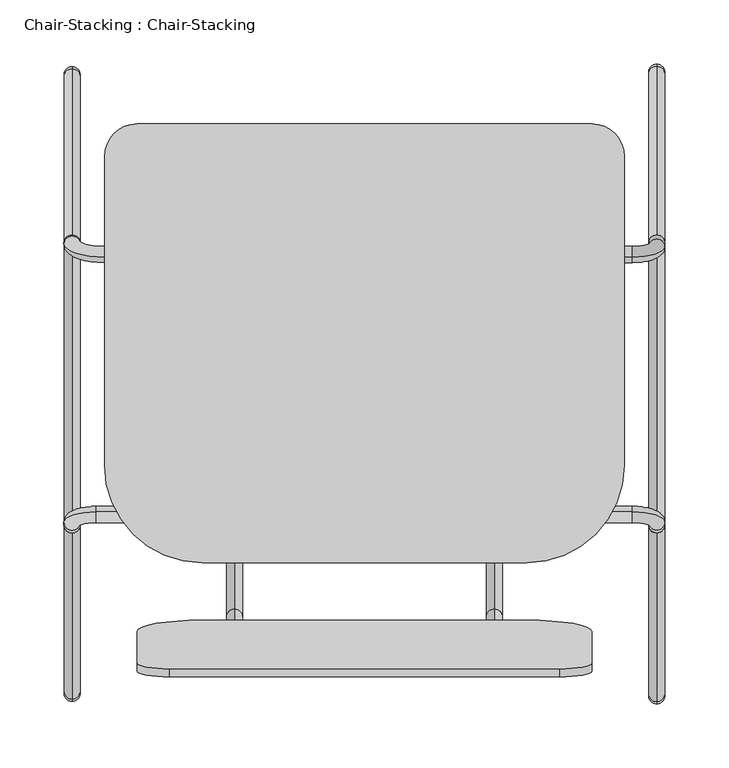
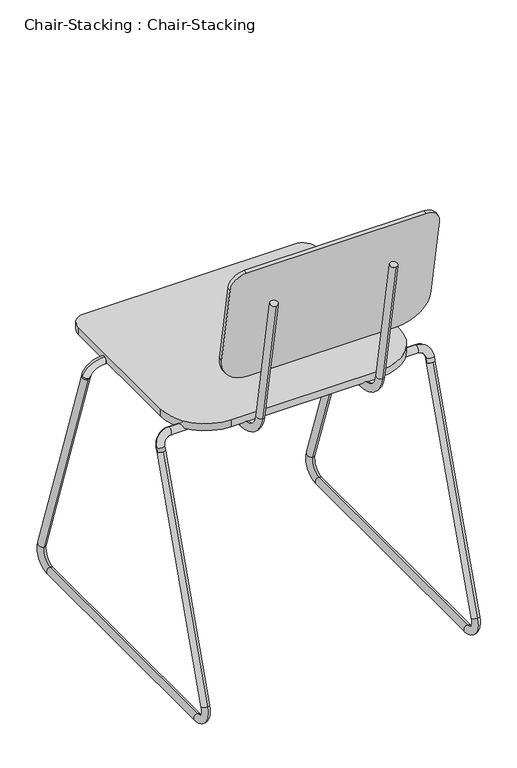
"""IFC4 building model written with IfcOpenShell, lengths in millimetres: furniture geometry, Chair-Stacking : Chair-Stacking."""

import ifcopenshell
import ifcopenshell.guid

model = None  # the IFC model being written
_history = None  # IfcOwnerHistory: only IFC2X3 demands one
_inside = {}  # id of a spatial element -> (the spatial element, [elements in it])
_under = {}  # id of a project, library or spatial element -> (it, [spatial elements below it])
_declared = {}  # id of a project -> (the project, [libraries it declares])
_typed = {}  # id of a type object -> (the type object, [elements of that type])
_made_of = {}  # id of a material, layer set ... -> (it, [elements and type objects made of it])


def new_model(schema):
    """Start an empty IFC model of exactly this schema.

    Asked for "IFC4X3", IfcOpenShell would pick the latest addendum, in which some entities
    have other attributes; the version numbers below select the first issue.
    IFC2X3 requires an IfcOwnerHistory on every rooted entity: one is made here for all.
    """
    global model, _history
    if schema == "IFC4X3":
        model = ifcopenshell.file(schema_version=(4, 3, 0, 0))
    else:
        model = ifcopenshell.file(schema=schema)
    _inside.clear()
    _under.clear()
    _declared.clear()
    _typed.clear()
    _made_of.clear()
    _history = None
    if model.schema == "IFC2X3":
        org = make("IfcOrganization", Name="unknown")
        user = make(
            "IfcPersonAndOrganization",
            ThePerson=make("IfcPerson", FamilyName="unknown"),
            TheOrganization=org,
        )
        app = make(
            "IfcApplication",
            ApplicationDeveloper=org,
            Version="unknown",
            ApplicationFullName="unknown",
            ApplicationIdentifier="unknown",
        )
        _history = make(
            "IfcOwnerHistory",
            OwningUser=user,
            OwningApplication=app,
            ChangeAction="ADDED",
            CreationDate=0,
        )
    return model


def make(cls, **values):
    """One entity of the class cls with the attributes given. An attribute that is None is left unset."""
    return model.create_entity(
        cls, **{name: value for name, value in values.items() if value is not None}
    )


def rooted(cls, **values):
    """An entity with a GlobalId (a new one), such as an element, a storey or a relation."""
    return make(cls, GlobalId=ifcopenshell.guid.new(), OwnerHistory=_history, **values)


def si_unit(unit_type, name, prefix=None):
    """IfcSIUnit, for example si_unit("LENGTHUNIT", "METRE", prefix="MILLI")."""
    return make("IfcSIUnit", UnitType=unit_type, Prefix=prefix, Name=name)


def assignment(units):
    """IfcUnitAssignment: the units of a project."""
    return None if units is None else make("IfcUnitAssignment", Units=units)


def point(xyz):
    """IfcCartesianPoint."""
    return None if xyz is None else make("IfcCartesianPoint", Coordinates=xyz)


def direction(xyz):
    """IfcDirection."""
    return None if xyz is None else make("IfcDirection", DirectionRatios=xyz)


def frame(location, z_axis=None, x_axis=None):
    """IfcAxis2Placement3D, a coordinate frame: its origin and axes. An axis left out is left unset."""
    return make(
        "IfcAxis2Placement3D",
        Location=point(location),
        Axis=direction(z_axis),
        RefDirection=direction(x_axis),
    )


def frame_2d(location, x_axis=None):
    """IfcAxis2Placement2D, a coordinate frame in the plane: its origin and x axis."""
    return make(
        "IfcAxis2Placement2D", Location=point(location), RefDirection=direction(x_axis)
    )


def origin():
    """The frame at (0, 0, 0) with its axes left unset."""
    return frame((0.0, 0.0, 0.0))


def place(relative_to, where):
    """IfcLocalPlacement: puts the frame where relative to a parent placement (None: the world)."""
    return make(
        "IfcLocalPlacement", PlacementRelTo=relative_to, RelativePlacement=where
    )


def context(
    kind, dimensions, precision=None, world=None, true_north=None, identifier=None
):
    """IfcGeometricRepresentationContext, for example the 3D "Model" context."""
    return make(
        "IfcGeometricRepresentationContext",
        ContextIdentifier=identifier,
        ContextType=kind,
        CoordinateSpaceDimension=dimensions,
        Precision=precision,
        WorldCoordinateSystem=world,
        TrueNorth=true_north,
    )


def project(units=None, contexts=None):
    """IfcProject with its units and contexts."""
    return rooted(
        "IfcProject",
        Name="project",
        RepresentationContexts=contexts,
        UnitsInContext=assignment(units),
    )


def spatial(cls, under=None, at=None, **own):
    """A site, building, storey or space (cls), placed at a placement, below another one or the project."""
    s = rooted(cls, ObjectPlacement=at, **own)
    if under is not None:
        _under.setdefault(under.id(), (under, []))[1].append(s)
    return s


def polyline(points):
    """IfcPolyline through the points."""
    return make("IfcPolyline", Points=[point(p) for p in points])


def circle_curve(where, radius):
    """IfcCircle in the frame where."""
    return make("IfcCircle", Position=where, Radius=radius)


def ellipse_curve(where, semi_axis1, semi_axis2):
    """IfcEllipse in the frame where."""
    return make(
        "IfcEllipse", Position=where, SemiAxis1=semi_axis1, SemiAxis2=semi_axis2
    )


def trimmed(basis, trim1, trim2, sense, master):
    """IfcTrimmedCurve: the piece of a basis curve between two trims."""
    return make(
        "IfcTrimmedCurve",
        BasisCurve=basis,
        Trim1=trim1,
        Trim2=trim2,
        SenseAgreement=sense,
        MasterRepresentation=master,
    )


def segment(curve, same_sense, transition):
    """IfcCompositeCurveSegment."""
    return make(
        "IfcCompositeCurveSegment",
        Transition=transition,
        SameSense=same_sense,
        ParentCurve=curve,
    )


def composite_curve(segments, self_intersect=None):
    """IfcCompositeCurve: segments joined end to end."""
    return make("IfcCompositeCurve", Segments=segments, SelfIntersect=self_intersect)


def outline(outer, holes=None, kind="AREA"):
    """IfcArbitraryClosedProfileDef: a profile drawn as a closed curve; with holes, ...WithVoids."""
    if holes is None:
        return make("IfcArbitraryClosedProfileDef", ProfileType=kind, OuterCurve=outer)
    return make(
        "IfcArbitraryProfileDefWithVoids",
        ProfileType=kind,
        OuterCurve=outer,
        InnerCurves=holes,
    )


def extrude(swept, where, along, depth):
    """IfcExtrudedAreaSolid: the profile swept, set in the frame where, extruded along a direction by depth."""
    return make(
        "IfcExtrudedAreaSolid",
        SweptArea=swept,
        Position=where,
        ExtrudedDirection=direction(along),
        Depth=depth,
    )


def shape(context_of_items, identifier, shape_type, items):
    """IfcShapeRepresentation: the items that make up one representation, for example the "Body"."""
    return make(
        "IfcShapeRepresentation",
        ContextOfItems=context_of_items,
        RepresentationIdentifier=identifier,
        RepresentationType=shape_type,
        Items=items,
    )


def source(mapping_origin, context_of_items, identifier, shape_type, items):
    """IfcRepresentationMap: a shape defined once, which mapped items show again and again."""
    return make(
        "IfcRepresentationMap",
        MappingOrigin=mapping_origin,
        MappedRepresentation=shape(context_of_items, identifier, shape_type, items),
    )


def transform(
    local_origin,
    x_axis=None,
    y_axis=None,
    z_axis=None,
    scale=None,
    scale2=None,
    scale3=None,
    uniform=True,
):
    """IfcCartesianTransformationOperator3D, or its non-uniform kind. x_axis, y_axis, z_axis: its Axis1, 2, 3."""
    if uniform:
        return make(
            "IfcCartesianTransformationOperator3D",
            Axis1=direction(x_axis),
            Axis2=direction(y_axis),
            LocalOrigin=point(local_origin),
            Scale=scale,
            Axis3=direction(z_axis),
        )
    return make(
        "IfcCartesianTransformationOperator3DnonUniform",
        Axis1=direction(x_axis),
        Axis2=direction(y_axis),
        LocalOrigin=point(local_origin),
        Scale=scale,
        Axis3=direction(z_axis),
        Scale2=scale2,
        Scale3=scale3,
    )


def mapped(mapping_source, mapping_target):
    """IfcMappedItem: shows the shape of a source again, moved by a transform."""
    return make(
        "IfcMappedItem", MappingSource=mapping_source, MappingTarget=mapping_target
    )


def made_of(thing, what):
    """Note that an element or type object is made of a material, layer set ...; save() writes the relation."""
    if what is not None:
        _made_of.setdefault(what.id(), (what, []))[1].append(thing)
    return thing


def element(
    cls,
    number,
    at=None,
    inside=None,
    cuts=None,
    type_object=None,
    material=None,
    context=None,
    identifier="Body",
    shape_type=None,
    held_by="IfcProductDefinitionShape",
    body=None,
    shapes=None,
    **own,
):
    """One element of the class cls, such as IfcWall. Its Tag is "e" and its number.

    at: its placement. inside: the storey or other place that contains it. cuts: it is an
    opening in that element (IfcRelVoidsElement). A single representation is given by context,
    identifier, shape_type and body (its items); several are given by shapes. held_by: the class
    of the entity that holds the representations. save() writes the other relations.
    """
    e = rooted(cls, Tag="e%d" % number, ObjectPlacement=at, **own)
    if body is not None:
        shapes = [shape(context, identifier, shape_type, body)]
    if shapes is not None:
        e.Representation = make(held_by, Representations=shapes)
    if inside is not None:
        _inside.setdefault(inside.id(), (inside, []))[1].append(e)
    if cuts is not None:
        rooted(
            "IfcRelVoidsElement", RelatingBuildingElement=cuts, RelatedOpeningElement=e
        )
    if type_object is not None:
        _typed.setdefault(type_object.id(), (type_object, []))[1].append(e)
    return made_of(e, material)


def aggregate(whole, parts):
    """IfcRelAggregates: a whole, such as a stair, and the parts it consists of."""
    return rooted("IfcRelAggregates", RelatingObject=whole, RelatedObjects=parts)


def save(model, path):
    """Write the relations noted so far, then the file.

    IfcRelAggregates (storeys below a building ...), IfcRelContainedInSpatialStructure (elements
    in a storey), IfcRelDefinesByType, IfcRelAssociatesMaterial and IfcRelDeclares: one each for
    every whole, place, type object, material and project.
    """
    for whole, parts in _under.values():
        aggregate(whole, parts)
    for where, things in _inside.values():
        rooted(
            "IfcRelContainedInSpatialStructure",
            RelatedElements=things,
            RelatingStructure=where,
        )
    for kind, things in _typed.values():
        rooted("IfcRelDefinesByType", RelatedObjects=things, RelatingType=kind)
    for what, things in _made_of.values():
        rooted("IfcRelAssociatesMaterial", RelatedObjects=things, RelatingMaterial=what)
    for by, libraries in _declared.values():
        rooted("IfcRelDeclares", RelatingContext=by, RelatedDefinitions=libraries)
    model.write(path)


def plane_surface(at):
    """IfcPlane: the flat surface through the origin of the frame at, square to its z axis."""
    return make("IfcPlane", Position=at)


def cylinder_surface(at, radius):
    """IfcCylindricalSurface: all points at the distance radius from the z axis of the frame at."""
    return make("IfcCylindricalSurface", Position=at, Radius=radius)


def revolved_surface(curve, axis_point, axis_direction):
    """IfcSurfaceOfRevolution: the curve turned about the line through axis_point along axis_direction."""
    return make(
        "IfcSurfaceOfRevolution",
        SweptCurve=make("IfcArbitraryOpenProfileDef", ProfileType="CURVE", Curve=curve),
        AxisPosition=make("IfcAxis1Placement", Location=point(axis_point), Axis=direction(axis_direction)),
    )


def advanced_brep(points, edges, surfaces, faces):
    """IfcAdvancedBrep: a solid bounded by faces that lie on surfaces and meet in shared edges.

    An edge is (start, end): straight between two places in points (the first is 0);
    or (start, end, curve); or (start, end, curve, False) where it runs against its curve.
    A face is (place in surfaces, loops), or (place, loops, False) where it looks against
    its surface's normal. A loop lists edges by number (the first is 1), with a minus sign
    where the edge is run from its end to its start. The first loop is the outer one.
    """
    corners = [point(p) for p in points]
    vertices = [make("IfcVertexPoint", VertexGeometry=c) for c in corners]
    made = []
    for start, end, *more in edges:
        made.append(
            make(
                "IfcEdgeCurve",
                EdgeStart=vertices[start],
                EdgeEnd=vertices[end],
                EdgeGeometry=more[0] if more else make("IfcPolyline", Points=[corners[start], corners[end]]),
                SameSense=more[1] if len(more) > 1 else True,
            )
        )
    hull = []
    for where, loops, *sense in faces:
        bounds = []
        for j, loop in enumerate(loops):
            ring = [make("IfcOrientedEdge", EdgeElement=made[abs(k) - 1], Orientation=k > 0) for k in loop]
            bounds.append(
                make(
                    "IfcFaceOuterBound" if j == 0 else "IfcFaceBound",
                    Bound=make("IfcEdgeLoop", EdgeList=ring),
                    Orientation=True,
                )
            )
        hull.append(make("IfcAdvancedFace", Bounds=bounds, FaceSurface=surfaces[where], SameSense=sense[0] if sense else True))
    return make("IfcAdvancedBrep", Outer=make("IfcClosedShell", CfsFaces=hull))


def chair_stacking_chair_stacking_76f41a28(model_context):
    return source(origin(), model_context, "Body", "SolidModel", [
        advanced_brep(
        [(-280.6491803, 213.2656675, 431.8), (-280.6491803, 213.2656675, 444.5), (-280.6491803, -23.0277124, 431.8), (-280.6491803, -23.0277124, 444.5), (-280.6491803, -66.802417, 481.2313385), (-280.6491803, -79.3094755, 479.0260066), (-280.6491803, -119.2282049, 705.4163709), (-280.6491803, -106.7211464, 707.6217027)],
        [
            (0, 1, circle_curve(frame((-280.6491803, 213.2656675, 438.15), z_axis=(0.0, 1.0, 0.0), x_axis=(0.0, 0.0, 1.0)), 6.35)),
            (1, 0, circle_curve(frame((-280.6491803, 213.2656675, 438.15), z_axis=(0.0, 1.0, 0.0), x_axis=(0.0, 0.0, 1.0)), 6.35)),
            (0, 2),
            (2, 3, circle_curve(frame((-280.6491803, -23.0277124, 438.15), z_axis=(0.0, 1.0, 0.0), x_axis=(0.0, 0.0, 1.0)), 6.35)),
            (3, 1),
            (3, 2, circle_curve(frame((-280.6491803, -23.0277124, 438.15), z_axis=(0.0, 1.0, 0.0), x_axis=(0.0, 0.0, 1.0)), 6.35)),
            (4, 3, circle_curve(frame((-280.6491803, -23.0277124, 488.95), z_axis=(1.0, 0.0, 0.0), x_axis=(0.0, 0.0, -1.0)), 44.45)),
            (2, 5, circle_curve(frame((-280.6491803, -23.0277124, 488.95), z_axis=(-1.0, 0.0, 0.0), x_axis=(0.0, 0.0, -1.0)), 57.15)),
            (5, 4, circle_curve(frame((-280.6491803, -73.0559463, 480.1286726), z_axis=(0.0, 0.17364817766693444, -0.9848077530122074), x_axis=(0.0, 0.9848077530122074, 0.17364817766693444)), 6.35)),
            (4, 5, circle_curve(frame((-280.6491803, -73.0559463, 480.1286726), z_axis=(0.0, 0.17364817766693444, -0.9848077530122074), x_axis=(0.0, 0.9848077530122074, 0.17364817766693444)), 6.35)),
            (6, 7, circle_curve(frame((-280.6491803, -112.9746757, 706.5190368), z_axis=(0.0, -0.1736481776669348, 0.9848077530122074), x_axis=(0.0, 0.9848077530122074, 0.1736481776669348)), 6.35)),
            (7, 6, circle_curve(frame((-280.6491803, -112.9746757, 706.5190368), z_axis=(0.0, -0.1736481776669348, 0.9848077530122074), x_axis=(0.0, 0.9848077530122074, 0.1736481776669348)), 6.35)),
            (5, 6),
            (7, 4),
        ],
        [
            plane_surface(frame((-286.9991803, 213.2656675, 438.15), z_axis=(0.0, 1.0, 0.0), x_axis=(0.0, 0.0, -1.0))),
            cylinder_surface(frame((-280.6491803, 213.2656675, 438.15), z_axis=(0.0, 1.0, 0.0), x_axis=(0.0, 0.0, 1.0)), 6.35),
            revolved_surface(trimmed(ellipse_curve(frame((-280.6491803, -23.0277124, 438.15), z_axis=(0.0, 1.0, 0.0), x_axis=(0.0, 0.0, 1.0)), 6.35, 6.35), [point((-280.6491803, -23.0277124, 431.8))], [point((-280.6491803, -23.0277124, 444.5))], True, "CARTESIAN"), (-280.6491803, -23.0277124, 488.95), (-1.0, 0.0, 0.0)),
            revolved_surface(trimmed(ellipse_curve(frame((-280.6491803, -23.0277124, 438.15), z_axis=(0.0, 1.0, 0.0), x_axis=(0.0, 0.0, 1.0)), 6.35, 6.35), [point((-280.6491803, -23.0277124, 444.5))], [point((-280.6491803, -23.0277124, 431.8))], True, "CARTESIAN"), (-280.6491803, -23.0277124, 488.95), (-1.0, 0.0, 0.0)),
            plane_surface(frame((-280.6491803, -119.2282049, 705.4163709), z_axis=(0.0, -0.17364817766692842, 0.9848077530122085), x_axis=(1.0, 0.0, 0.0))),
            cylinder_surface(frame((-280.6491803, -73.0559463, 480.1286726), z_axis=(0.0, 0.1736481776669348, -0.9848077530122074), x_axis=(0.0, 0.9848077530122074, 0.1736481776669348)), 6.35),
        ],
        [
            (0, [[1, 2]]),
            (1, [[-1, 3, 4, 5]]),
            (1, [[-2, -5, 6, -3]]),
            (2, [[7, -4, 8, 9]]),
            (3, [[-8, -6, -7, 10]]),
            (4, [[11, 12]]),
            (5, [[-9, 13, -12, 14]]),
            (5, [[-10, -14, -11, -13]]),
        ],
    ),
        advanced_brep(
        [(-77.4491803, 213.2656675, 431.8), (-77.4491803, 213.2656675, 444.5), (-77.4491803, -23.0277124, 431.8), (-77.4491803, -23.0277124, 444.5), (-77.4491803, -66.802417, 481.2313385), (-77.4491803, -79.3094755, 479.0260066), (-77.4491803, -118.9339087, 703.7473341), (-77.4491803, -106.4268502, 705.9526659)],
        [
            (0, 1, circle_curve(frame((-77.4491803, 213.2656675, 438.15), z_axis=(0.0, 1.0, 0.0), x_axis=(0.0, 0.0, 1.0)), 6.35)),
            (1, 0, circle_curve(frame((-77.4491803, 213.2656675, 438.15), z_axis=(0.0, 1.0, 0.0), x_axis=(0.0, 0.0, 1.0)), 6.35)),
            (0, 2),
            (2, 3, circle_curve(frame((-77.4491803, -23.0277124, 438.15), z_axis=(0.0, 1.0, 0.0), x_axis=(0.0, 0.0, 1.0)), 6.35)),
            (3, 1),
            (3, 2, circle_curve(frame((-77.4491803, -23.0277124, 438.15), z_axis=(0.0, 1.0, 0.0), x_axis=(0.0, 0.0, 1.0)), 6.35)),
            (4, 3, circle_curve(frame((-77.4491803, -23.0277124, 488.95), z_axis=(1.0, 0.0, 0.0), x_axis=(0.0, 0.0, -1.0)), 44.45)),
            (2, 5, circle_curve(frame((-77.4491803, -23.0277124, 488.95), z_axis=(-1.0, 0.0, 0.0), x_axis=(0.0, 0.0, -1.0)), 57.15)),
            (5, 4, circle_curve(frame((-77.4491803, -73.0559463, 480.1286726), z_axis=(0.0, 0.1736481776669385, -0.9848077530122066), x_axis=(0.0, 0.9848077530122066, 0.1736481776669385)), 6.35)),
            (4, 5, circle_curve(frame((-77.4491803, -73.0559463, 480.1286726), z_axis=(0.0, 0.1736481776669372, -0.9848077530122068), x_axis=(0.0, 0.9848077530122068, 0.1736481776669372)), 6.35)),
            (6, 7, circle_curve(frame((-77.4491803, -112.6803794, 704.85), z_axis=(0.0, -0.17364817766693896, 0.9848077530122066), x_axis=(0.0, 0.9848077530122066, 0.17364817766693896)), 6.35)),
            (7, 6, circle_curve(frame((-77.4491803, -112.6803794, 704.85), z_axis=(0.0, -0.17364817766693896, 0.9848077530122066), x_axis=(0.0, 0.9848077530122066, 0.17364817766693896)), 6.35)),
            (5, 6),
            (7, 4),
        ],
        [
            plane_surface(frame((-83.7991803, 213.2656675, 438.15), z_axis=(0.0, 1.0, 0.0), x_axis=(0.0, 0.0, -1.0))),
            cylinder_surface(frame((-77.4491803, 213.2656675, 438.15), z_axis=(0.0, 1.0, 0.0), x_axis=(0.0, 0.0, 1.0)), 6.35),
            revolved_surface(trimmed(ellipse_curve(frame((-77.4491803, -23.0277124, 438.15), z_axis=(0.0, 1.0, 0.0), x_axis=(0.0, 0.0, 1.0)), 6.35, 6.35), [point((-77.4491803, -23.0277124, 431.8))], [point((-77.4491803, -23.0277124, 444.5))], True, "CARTESIAN"), (-77.4491803, -23.0277124, 488.95), (-1.0, 0.0, 0.0)),
            revolved_surface(trimmed(ellipse_curve(frame((-77.4491803, -23.0277124, 438.15), z_axis=(0.0, 1.0, 0.0), x_axis=(0.0, 0.0, 1.0)), 6.35, 6.35), [point((-77.4491803, -23.0277124, 444.5))], [point((-77.4491803, -23.0277124, 431.8))], True, "CARTESIAN"), (-77.4491803, -23.0277124, 488.95), (-1.0, 0.0, 0.0)),
            plane_surface(frame((-77.4491803, -118.9339087, 703.7473341), z_axis=(0.0, -0.17364817766692892, 0.9848077530122084), x_axis=(1.0, 0.0, 0.0))),
            cylinder_surface(frame((-77.4491803, -73.0559463, 480.1286726), z_axis=(0.0, 0.17364817766693896, -0.9848077530122066), x_axis=(0.0, 0.9848077530122066, 0.17364817766693896)), 6.35),
        ],
        [
            (0, [[1, 2]]),
            (1, [[-1, 3, 4, 5]]),
            (1, [[-2, -5, 6, -3]]),
            (2, [[7, -4, 8, 9]]),
            (3, [[-8, -6, -7, 10]]),
            (4, [[11, 12]]),
            (5, [[-9, 13, -12, 14]]),
            (5, [[-10, -14, -11, -13]]),
        ],
    ),
        extrude(outline(composite_curve([segment(trimmed(circle_curve(frame_2d((-1.2491803, 286.7314636)), 25.4), [point((-1.2491803, 312.1314636))], [point((24.1508197, 286.7314636))], False, "CARTESIAN"), True, "CONTINUOUS"), segment(polyline([(24.1508197, 286.7314636), (24.1508197, 45.4314636)]), True, "CONTINUOUS"), segment(trimmed(circle_curve(frame_2d((-52.0491803, 45.4314636)), 76.2), [point((24.1508197, 45.4314636))], [point((-52.0491803, -30.7685364))], False, "CARTESIAN"), True, "CONTINUOUS"), segment(polyline([(-52.0491803, -30.7685364), (-306.0491803, -30.7685364)]), True, "CONTINUOUS"), segment(trimmed(circle_curve(frame_2d((-306.0491803, 45.4314636)), 76.2), [point((-306.0491803, -30.7685364))], [point((-382.2491803, 45.4314636))], False, "CARTESIAN"), True, "CONTINUOUS"), segment(polyline([(-382.2491803, 45.4314636), (-382.2491803, 286.7314636)]), True, "CONTINUOUS"), segment(trimmed(circle_curve(frame_2d((-356.8491803, 286.7314636)), 25.4), [point((-382.2491803, 286.7314636))], [point((-356.8491803, 312.1314636))], False, "CARTESIAN"), True, "CONTINUOUS"), segment(polyline([(-356.8491803, 312.1314636), (-1.2491803, 312.1314636)]), True, "CONTINUOUS")], self_intersect=False)), frame((0.0, 0.0, 444.5), z_axis=(0.0, 0.0, 1.0), x_axis=(1.0, 0.0, 0.0)), (0.0, 0.0, 1.0), 12.7),
        extrude(outline(composite_curve([segment(polyline([(-304.8, 0.0), (0.0, 0.0)]), True, "CONTINUOUS"), segment(trimmed(circle_curve(frame_2d((0.0, -25.4)), 25.4), [point((0.0, 0.0))], [point((25.4, -25.4))], False, "CARTESIAN"), True, "CONTINUOUS"), segment(polyline([(25.4, -25.4), (25.4, -168.3013626)]), True, "CONTINUOUS"), segment(trimmed(circle_curve(frame_2d((-25.4, -168.3013626)), 50.8), [point((25.4, -168.3013626))], [point((-25.4, -219.1013626))], False, "CARTESIAN"), True, "CONTINUOUS"), segment(polyline([(-25.4, -219.1013626), (-279.4, -219.1013626)]), True, "CONTINUOUS"), segment(trimmed(circle_curve(frame_2d((-279.4, -168.3013626)), 50.8), [point((-279.4, -219.1013626))], [point((-330.2, -168.3013626))], False, "CARTESIAN"), True, "CONTINUOUS"), segment(polyline([(-330.2, -168.3013626), (-330.2, -25.4)]), True, "CONTINUOUS"), segment(trimmed(circle_curve(frame_2d((-304.8, -25.4)), 25.4), [point((-330.2, -25.4))], [point((-304.8, 0.0))], False, "CARTESIAN"), True, "CONTINUOUS")], self_intersect=False)), frame((-331.4491803, -119.9531376, 782.6640535), z_axis=(0.0, 0.9848077530122084, 0.17364817766692858), x_axis=(-1.0, 0.0, 0.0)), (0.0, 0.0, 1.0), 6.35),
        advanced_brep(
        [(55.9008197, 219.2327758, 419.1211728), (43.2008197, 219.2327758, 419.1211728), (55.9008197, 216.3017292, 427.6700586), (43.2008197, 216.3017292, 427.6700586), (30.5008197, 212.1828103, 439.6835721), (30.5008197, 208.0638914, 451.6970857), (-382.2491803, 208.0638914, 451.6970857), (-382.2491803, 212.1828103, 439.6835721), (-401.2991803, 218.3611887, 421.6633019), (-413.9991803, 218.3611887, 421.6633019), (-413.9991803, 219.2424531, 419.0929473), (-401.2991803, 219.2424531, 419.0929473)],
        [
            (0, 1, circle_curve(frame((49.5508197, 219.2327758, 419.1211728), z_axis=(0.0, 0.32432432432432967, -0.9459459459459442), x_axis=(-1.0, 0.0, 0.0)), 6.35)),
            (1, 0, circle_curve(frame((49.5508197, 219.2327758, 419.1211728), z_axis=(0.0, 0.32432432432432967, -0.9459459459459442), x_axis=(-1.0, 0.0, 0.0)), 6.35)),
            (0, 2),
            (2, 3, circle_curve(frame((49.5508197, 216.3017292, 427.6700586), z_axis=(0.0, 0.32432432432432967, -0.9459459459459442), x_axis=(-1.0, 0.0, 0.0)), 6.35)),
            (3, 1),
            (3, 2, circle_curve(frame((49.5508197, 216.3017292, 427.6700586), z_axis=(0.0, 0.32432432432432967, -0.9459459459459442), x_axis=(-1.0, 0.0, 0.0)), 6.35)),
            (4, 3, circle_curve(frame((30.5008197, 216.3017292, 427.6700586), z_axis=(0.0, 0.9459459459459447, 0.3243243243243281), x_axis=(1.0, 0.0, 0.0)), 12.7)),
            (2, 5, circle_curve(frame((30.5008197, 216.3017292, 427.6700586), z_axis=(0.0, -0.9459459459459447, -0.3243243243243281), x_axis=(1.0, 0.0, 0.0)), 25.4)),
            (5, 4, circle_curve(frame((30.5008197, 210.1233509, 445.6903289), z_axis=(1.0, 0.0, 0.0), x_axis=(0.0, 0.32432432432432745, -0.9459459459459449)), 6.35)),
            (4, 5, circle_curve(frame((30.5008197, 210.1233509, 445.6903289), z_axis=(1.0, 0.0, 0.0), x_axis=(0.0, 0.32432432432432745, -0.9459459459459449)), 6.35)),
            (5, 6),
            (6, 7, circle_curve(frame((-382.2491803, 210.1233509, 445.6903289), z_axis=(1.0, 0.0, 0.0), x_axis=(0.0, 0.32432432432432745, -0.9459459459459449)), 6.35)),
            (7, 4),
            (7, 6, circle_curve(frame((-382.2491803, 210.1233509, 445.6903289), z_axis=(1.0, 0.0, 0.0), x_axis=(0.0, 0.32432432432432745, -0.9459459459459449)), 6.35)),
            (8, 7, circle_curve(frame((-382.2491803, 218.3611887, 421.6633019), z_axis=(0.0, 0.9459459459459447, 0.3243243243243281), x_axis=(0.0, -0.3243243243243281, 0.9459459459459447)), 19.05)),
            (6, 9, circle_curve(frame((-382.2491803, 218.3611887, 421.6633019), z_axis=(0.0, -0.9459459459459447, -0.3243243243243281), x_axis=(0.0, -0.3243243243243281, 0.9459459459459447)), 31.75)),
            (9, 8, circle_curve(frame((-407.6491803, 218.3611887, 421.6633019), z_axis=(0.0, -0.324324324324328, 0.9459459459459447), x_axis=(1.0000000000000002, 0.0, 0.0)), 6.35)),
            (8, 9, circle_curve(frame((-407.6491803, 218.3611887, 421.6633019), z_axis=(0.0, -0.324324324324328, 0.9459459459459447), x_axis=(1.0000000000000002, 0.0, 0.0)), 6.35)),
            (10, 11, circle_curve(frame((-407.6491803, 219.2424531, 419.0929473), z_axis=(0.0, 0.32432432432432784, -0.9459459459459449), x_axis=(1.0, 0.0, 0.0)), 6.35)),
            (11, 10, circle_curve(frame((-407.6491803, 219.2424531, 419.0929473), z_axis=(0.0, 0.32432432432432784, -0.9459459459459449), x_axis=(1.0, 0.0, 0.0)), 6.35)),
            (9, 10),
            (11, 8),
        ],
        [
            plane_surface(frame((49.5508197, 213.226019, 417.0617133), z_axis=(0.0, 0.32432432432433117, -0.9459459459459437), x_axis=(1.0, 0.0, 0.0))),
            cylinder_surface(frame((49.5508197, 219.2327758, 419.1211728), z_axis=(0.0, 0.32432432432432967, -0.9459459459459442), x_axis=(-1.0, 0.0, 0.0)), 6.35),
            revolved_surface(trimmed(ellipse_curve(frame((49.5508197, 216.3017292, 427.6700586), z_axis=(0.0, 0.32432432432432823, -0.9459459459459447), x_axis=(-1.0, 0.0, 0.0)), 6.35, 6.35), [point((55.9008197, 216.3017292, 427.6700586))], [point((43.2008197, 216.3017292, 427.6700586))], True, "CARTESIAN"), (30.5008197, 216.3017292, 427.6700586), (0.0, -0.9459459459459447, -0.3243243243243281)),
            revolved_surface(trimmed(ellipse_curve(frame((49.5508197, 216.3017292, 427.6700586), z_axis=(0.0, 0.32432432432432823, -0.9459459459459447), x_axis=(-1.0, 0.0, 0.0)), 6.35, 6.35), [point((43.2008197, 216.3017292, 427.6700586))], [point((55.9008197, 216.3017292, 427.6700586))], True, "CARTESIAN"), (30.5008197, 216.3017292, 427.6700586), (0.0, -0.9459459459459447, -0.3243243243243281)),
            cylinder_surface(frame((30.5008197, 210.1233509, 445.6903289), z_axis=(1.0, 0.0, 0.0), x_axis=(0.0, 0.32432432432432745, -0.9459459459459449)), 6.35),
            revolved_surface(trimmed(ellipse_curve(frame((-382.2491803, 210.1233509, 445.6903289), z_axis=(1.0000000000000002, 0.0, 0.0), x_axis=(0.0, 0.3243243243243276, -0.9459459459459448)), 6.35, 6.35), [point((-382.2491803, 208.0638914, 451.6970857))], [point((-382.2491803, 212.1828103, 439.6835721))], True, "CARTESIAN"), (-382.2491803, 218.3611887, 421.6633019), (0.0, -0.9459459459459447, -0.3243243243243281)),
            revolved_surface(trimmed(ellipse_curve(frame((-382.2491803, 210.1233509, 445.6903289), z_axis=(1.0000000000000002, 0.0, 0.0), x_axis=(0.0, 0.3243243243243276, -0.9459459459459448)), 6.35, 6.35), [point((-382.2491803, 212.1828103, 439.6835721))], [point((-382.2491803, 208.0638914, 451.6970857))], True, "CARTESIAN"), (-382.2491803, 218.3611887, 421.6633019), (0.0, -0.9459459459459447, -0.3243243243243281)),
            plane_surface(frame((-407.6491803, 225.2492099, 421.1524068), z_axis=(0.0, 0.3243243243243264, -0.9459459459459453), x_axis=(1.0, 0.0, 0.0))),
            cylinder_surface(frame((-407.6491803, 218.3611887, 421.6633019), z_axis=(0.0, -0.3243243243243278, 0.9459459459459447), x_axis=(1.0, 0.0, 0.0)), 6.35),
        ],
        [
            (0, [[1, 2]]),
            (1, [[-1, 3, 4, 5]]),
            (1, [[-2, -5, 6, -3]]),
            (2, [[7, -4, 8, 9]]),
            (3, [[-8, -6, -7, 10]]),
            (4, [[-9, 11, 12, 13]]),
            (4, [[-10, -13, 14, -11]]),
            (5, [[15, -12, 16, 17]]),
            (6, [[-16, -14, -15, 18]]),
            (7, [[19, 20]]),
            (8, [[-17, 21, -20, 22]]),
            (8, [[-18, -22, -19, -21]]),
        ],
    ),
        advanced_brep(
        [(55.9008197, -1.3812406, 419.0879461), (43.2008197, -1.3812406, 419.0879461), (55.9008197, 0.7944914, 425.4338312), (43.2008197, 0.7944914, 425.4338312), (30.5008197, 4.9134104, 437.4473447), (30.5008197, 9.0323293, 449.4608582), (-388.5991803, 9.0323293, 449.4608582), (-388.5991803, 4.9134104, 437.4473447), (-401.2991803, 0.7944914, 425.4338312), (-413.9991803, 0.7944914, 425.4338312), (-413.9991803, -1.3997864, 419.0338542), (-401.2991803, -1.3997864, 419.0338542)],
        [
            (0, 1, circle_curve(frame((49.5508197, -1.3812406, 419.0879461), z_axis=(0.0, -0.32432432432432495, -0.9459459459459457), x_axis=(-1.0, 0.0, 0.0)), 6.35)),
            (1, 0, circle_curve(frame((49.5508197, -1.3812406, 419.0879461), z_axis=(0.0, -0.32432432432432495, -0.9459459459459457), x_axis=(-1.0, 0.0, 0.0)), 6.35)),
            (0, 2),
            (2, 3, circle_curve(frame((49.5508197, 0.7944914, 425.4338312), z_axis=(0.0, -0.32432432432432495, -0.9459459459459457), x_axis=(-1.0, 0.0, 0.0)), 6.35)),
            (3, 1),
            (3, 2, circle_curve(frame((49.5508197, 0.7944914, 425.4338312), z_axis=(0.0, -0.32432432432432495, -0.9459459459459457), x_axis=(-1.0, 0.0, 0.0)), 6.35)),
            (4, 3, circle_curve(frame((30.5008197, 0.7944914, 425.4338312), z_axis=(0.0, 0.9459459459459458, -0.3243243243243246), x_axis=(1.0, 0.0, 0.0)), 12.7)),
            (2, 5, circle_curve(frame((30.5008197, 0.7944914, 425.4338312), z_axis=(0.0, -0.9459459459459458, 0.3243243243243246), x_axis=(1.0, 0.0, 0.0)), 25.4)),
            (5, 4, circle_curve(frame((30.5008197, 6.9728698, 443.4541014), z_axis=(1.0, 0.0, 0.0), x_axis=(0.0, -0.3243243243243236, -0.9459459459459462)), 6.35)),
            (4, 5, circle_curve(frame((30.5008197, 6.9728698, 443.4541014), z_axis=(1.0, 0.0, 0.0), x_axis=(0.0, -0.3243243243243236, -0.9459459459459462)), 6.35)),
            (5, 6),
            (6, 7, circle_curve(frame((-388.5991803, 6.9728698, 443.4541014), z_axis=(1.0, 0.0, 0.0), x_axis=(0.0, -0.3243243243243236, -0.9459459459459462)), 6.35)),
            (7, 4),
            (7, 6, circle_curve(frame((-388.5991803, 6.9728698, 443.4541014), z_axis=(1.0, 0.0, 0.0), x_axis=(0.0, -0.3243243243243236, -0.9459459459459462)), 6.35)),
            (8, 7, circle_curve(frame((-388.5991803, 0.7944914, 425.4338312), z_axis=(0.0, 0.9459459459459458, -0.3243243243243246), x_axis=(0.0, 0.3243243243243246, 0.9459459459459458)), 12.7)),
            (6, 9, circle_curve(frame((-388.5991803, 0.7944914, 425.4338312), z_axis=(0.0, -0.9459459459459458, 0.3243243243243246), x_axis=(0.0, 0.3243243243243246, 0.9459459459459458)), 25.4)),
            (9, 8, circle_curve(frame((-407.6491803, 0.7944914, 425.4338312), z_axis=(0.0, 0.3243243243243247, 0.9459459459459458), x_axis=(1.0, 0.0, 0.0)), 6.35)),
            (8, 9, circle_curve(frame((-407.6491803, 0.7944914, 425.4338312), z_axis=(0.0, 0.3243243243243247, 0.9459459459459458), x_axis=(1.0, 0.0, 0.0)), 6.35)),
            (10, 11, circle_curve(frame((-407.6491803, -1.3997864, 419.0338542), z_axis=(0.0, -0.3243243243243242, -0.945945945945946), x_axis=(1.0, 0.0, 0.0)), 6.35)),
            (11, 10, circle_curve(frame((-407.6491803, -1.3997864, 419.0338542), z_axis=(0.0, -0.3243243243243242, -0.945945945945946), x_axis=(1.0, 0.0, 0.0)), 6.35)),
            (9, 10),
            (11, 8),
        ],
        [
            plane_surface(frame((49.5508197, -7.3879973, 421.1474055), z_axis=(0.0, -0.32432432432432273, -0.9459459459459466), x_axis=(1.0, 0.0, 0.0))),
            cylinder_surface(frame((49.5508197, -1.3812406, 419.0879461), z_axis=(0.0, -0.32432432432432495, -0.9459459459459457), x_axis=(-1.0, 0.0, 0.0)), 6.35),
            revolved_surface(trimmed(ellipse_curve(frame((49.5508197, 0.7944914, 425.4338312), z_axis=(0.0, -0.32432432432432456, -0.9459459459459458), x_axis=(-1.0, 0.0, 0.0)), 6.35, 6.35), [point((55.9008197, 0.7944914, 425.4338312))], [point((43.2008197, 0.7944914, 425.4338312))], True, "CARTESIAN"), (30.5008197, 0.7944914, 425.4338312), (0.0, -0.9459459459459458, 0.3243243243243246)),
            revolved_surface(trimmed(ellipse_curve(frame((49.5508197, 0.7944914, 425.4338312), z_axis=(0.0, -0.32432432432432456, -0.9459459459459458), x_axis=(-1.0, 0.0, 0.0)), 6.35, 6.35), [point((43.2008197, 0.7944914, 425.4338312))], [point((55.9008197, 0.7944914, 425.4338312))], True, "CARTESIAN"), (30.5008197, 0.7944914, 425.4338312), (0.0, -0.9459459459459458, 0.3243243243243246)),
            cylinder_surface(frame((30.5008197, 6.9728698, 443.4541014), z_axis=(1.0, 0.0, 0.0), x_axis=(0.0, -0.3243243243243236, -0.9459459459459462)), 6.35),
            revolved_surface(trimmed(ellipse_curve(frame((-388.5991803, 6.9728698, 443.4541014), z_axis=(1.0, 0.0, 0.0), x_axis=(0.0, -0.3243243243243236, -0.9459459459459462)), 6.35, 6.35), [point((-388.5991803, 9.0323293, 449.4608582))], [point((-388.5991803, 4.9134104, 437.4473447))], True, "CARTESIAN"), (-388.5991803, 0.7944914, 425.4338312), (0.0, -0.9459459459459458, 0.3243243243243246)),
            revolved_surface(trimmed(ellipse_curve(frame((-388.5991803, 6.9728698, 443.4541014), z_axis=(1.0, 0.0, 0.0), x_axis=(0.0, -0.3243243243243236, -0.9459459459459462)), 6.35, 6.35), [point((-388.5991803, 4.9134104, 437.4473447))], [point((-388.5991803, 9.0323293, 449.4608582))], True, "CARTESIAN"), (-388.5991803, 0.7944914, 425.4338312), (0.0, -0.9459459459459458, 0.3243243243243246)),
            plane_surface(frame((-407.6491803, 4.6069704, 416.9743947), z_axis=(0.0, -0.3243243243243226, -0.9459459459459466), x_axis=(1.0, 0.0, 0.0))),
            cylinder_surface(frame((-407.6491803, 0.7944914, 425.4338312), z_axis=(0.0, 0.3243243243243242, 0.945945945945946), x_axis=(1.0, 0.0, 0.0)), 6.35),
        ],
        [
            (0, [[1, 2]]),
            (1, [[-1, 3, 4, 5]]),
            (1, [[-2, -5, 6, -3]]),
            (2, [[7, -4, 8, 9]]),
            (3, [[-8, -6, -7, 10]]),
            (4, [[-9, 11, 12, 13]]),
            (4, [[-10, -13, 14, -11]]),
            (5, [[15, -12, 16, 17]]),
            (6, [[-16, -14, -15, 18]]),
            (7, [[19, 20]]),
            (8, [[-17, 21, -20, 22]]),
            (8, [[-18, -22, -19, -21]]),
        ],
    ),
        advanced_brep(
        [(-407.6491803, 225.2492099, 421.1524068), (-407.6491803, 213.2356963, 417.0334879), (-407.6491803, 355.2281045, 42.0472973), (-407.6491803, 343.214591, 37.9283784), (-407.6491803, 325.1943208, 12.7), (-407.6491803, 325.1943208, 0.0), (-407.6491803, -107.3313935, 0.0), (-407.6491803, -107.3313935, 12.7), (-407.6491803, -125.3516638, 37.9283784), (-407.6491803, -137.3651773, 42.0472973), (-407.6491803, -7.4065431, 421.0933136), (-407.6491803, 4.6069704, 416.9743947)],
        [
            (0, 1, circle_curve(frame((-407.6491803, 219.2424531, 419.0929473), z_axis=(0.0, -0.3243243243243311, 0.9459459459459437), x_axis=(0.0, -0.9459459459459437, -0.3243243243243311)), 6.35)),
            (1, 0, circle_curve(frame((-407.6491803, 219.2424531, 419.0929473), z_axis=(0.0, -0.3243243243243311, 0.9459459459459437), x_axis=(0.0, -0.9459459459459437, -0.3243243243243311)), 6.35)),
            (0, 2),
            (2, 3, circle_curve(frame((-407.6491803, 349.2213478, 39.9878378), z_axis=(0.0, -0.3243243243243311, 0.9459459459459437), x_axis=(0.0, -0.9459459459459437, -0.3243243243243311)), 6.35)),
            (3, 1),
            (3, 2, circle_curve(frame((-407.6491803, 349.2213478, 39.9878378), z_axis=(0.0, -0.3243243243243311, 0.9459459459459437), x_axis=(0.0, -0.9459459459459437, -0.3243243243243311)), 6.35)),
            (4, 3, circle_curve(frame((-407.6491803, 325.1943208, 31.75), z_axis=(1.0, 0.0, 0.0), x_axis=(0.0, 0.9459459459459434, 0.3243243243243317)), 19.05)),
            (2, 5, circle_curve(frame((-407.6491803, 325.1943208, 31.75), z_axis=(-1.0, 0.0, 0.0), x_axis=(0.0, 0.9459459459459434, 0.3243243243243317)), 31.75)),
            (5, 4, circle_curve(frame((-407.6491803, 325.1943208, 6.35), z_axis=(0.0, 1.0, 0.0), x_axis=(0.0, 0.0, 1.0)), 6.35)),
            (4, 5, circle_curve(frame((-407.6491803, 325.1943208, 6.35), z_axis=(0.0, 0.9999999999999999, 0.0), x_axis=(0.0, 0.0, 0.9999999999999999)), 6.35)),
            (5, 6),
            (6, 7, circle_curve(frame((-407.6491803, -107.3313935, 6.35), z_axis=(0.0, 1.0, 0.0), x_axis=(0.0, 0.0, 1.0)), 6.35)),
            (7, 4),
            (7, 6, circle_curve(frame((-407.6491803, -107.3313935, 6.35), z_axis=(0.0, 1.0, 0.0), x_axis=(0.0, 0.0, 1.0)), 6.35)),
            (8, 7, circle_curve(frame((-407.6491803, -107.3313935, 31.75), z_axis=(1.0, 0.0, 0.0), x_axis=(0.0, 0.0, -1.0)), 19.05)),
            (6, 9, circle_curve(frame((-407.6491803, -107.3313935, 31.75), z_axis=(-1.0, 0.0, 0.0), x_axis=(0.0, 0.0, -1.0)), 31.75)),
            (9, 8, circle_curve(frame((-407.6491803, -131.3584206, 39.9878378), z_axis=(0.0, -0.3243243243243189, -0.9459459459459478), x_axis=(0.0, 0.9459459459459478, -0.3243243243243189)), 6.35)),
            (8, 9, circle_curve(frame((-407.6491803, -131.3584206, 39.9878378), z_axis=(0.0, -0.3243243243243206, -0.9459459459459473), x_axis=(0.0, 0.9459459459459473, -0.3243243243243206)), 6.35)),
            (10, 11, circle_curve(frame((-407.6491803, -1.3997864, 419.0338542), z_axis=(0.0, 0.3243243243243217, 0.9459459459459468), x_axis=(0.0, 0.9459459459459468, -0.3243243243243217)), 6.35)),
            (11, 10, circle_curve(frame((-407.6491803, -1.3997864, 419.0338542), z_axis=(0.0, 0.3243243243243217, 0.9459459459459468), x_axis=(0.0, 0.9459459459459468, -0.3243243243243217)), 6.35)),
            (9, 10),
            (11, 8),
        ],
        [
            plane_surface(frame((-407.6491803, 225.2492099, 421.1524068), z_axis=(0.0, -0.32432432432432773, 0.9459459459459448), x_axis=(1.0, 0.0, 0.0))),
            cylinder_surface(frame((-407.6491803, 219.2424531, 419.0929473), z_axis=(0.0, -0.3243243243243311, 0.9459459459459437), x_axis=(0.0, -0.9459459459459437, -0.3243243243243311)), 6.35),
            revolved_surface(trimmed(ellipse_curve(frame((-407.6491803, 349.2213478, 39.9878378), z_axis=(0.0, -0.3243243243243347, 0.9459459459459424), x_axis=(0.0, -0.9459459459459424, -0.3243243243243347)), 6.35, 6.35), [point((-407.6491803, 355.2281045, 42.0472973))], [point((-407.6491803, 343.214591, 37.9283784))], True, "CARTESIAN"), (-407.6491803, 325.1943208, 31.75), (-1.0, 0.0, 0.0)),
            revolved_surface(trimmed(ellipse_curve(frame((-407.6491803, 349.2213478, 39.9878378), z_axis=(0.0, -0.3243243243243347, 0.9459459459459424), x_axis=(0.0, -0.9459459459459424, -0.3243243243243347)), 6.35, 6.35), [point((-407.6491803, 343.214591, 37.9283784))], [point((-407.6491803, 355.2281045, 42.0472973))], True, "CARTESIAN"), (-407.6491803, 325.1943208, 31.75), (-1.0, 0.0, 0.0)),
            cylinder_surface(frame((-407.6491803, 325.1943208, 6.35), z_axis=(0.0, 1.0, 0.0), x_axis=(0.0, 0.0, 1.0)), 6.35),
            revolved_surface(trimmed(ellipse_curve(frame((-407.6491803, -107.3313935, 6.35), z_axis=(0.0, 1.0, 0.0), x_axis=(0.0, 0.0, 1.0)), 6.35, 6.35), [point((-407.6491803, -107.3313935, 0.0))], [point((-407.6491803, -107.3313935, 12.7))], True, "CARTESIAN"), (-407.6491803, -107.3313935, 31.75), (-1.0, 0.0, 0.0)),
            revolved_surface(trimmed(ellipse_curve(frame((-407.6491803, -107.3313935, 6.35), z_axis=(0.0, 1.0, 0.0), x_axis=(0.0, 0.0, 1.0)), 6.35, 6.35), [point((-407.6491803, -107.3313935, 12.7))], [point((-407.6491803, -107.3313935, 0.0))], True, "CARTESIAN"), (-407.6491803, -107.3313935, 31.75), (-1.0, 0.0, 0.0)),
            plane_surface(frame((-407.6491803, -7.4065431, 421.0933136), z_axis=(0.0, 0.324324324324323, 0.9459459459459465), x_axis=(1.0, 0.0, 0.0))),
            cylinder_surface(frame((-407.6491803, -131.3584206, 39.9878378), z_axis=(0.0, -0.3243243243243217, -0.9459459459459468), x_axis=(0.0, 0.9459459459459468, -0.3243243243243217)), 6.35),
        ],
        [
            (0, [[1, 2]]),
            (1, [[-1, 3, 4, 5]]),
            (1, [[-2, -5, 6, -3]]),
            (2, [[7, -4, 8, 9]]),
            (3, [[-8, -6, -7, 10]]),
            (4, [[-9, 11, 12, 13]]),
            (4, [[-10, -13, 14, -11]]),
            (5, [[15, -12, 16, 17]]),
            (6, [[-16, -14, -15, 18]]),
            (7, [[19, 20]]),
            (8, [[-17, 21, -20, 22]]),
            (8, [[-18, -22, -19, -21]]),
        ],
    ),
        advanced_brep(
        [(49.5508197, 225.2597598, 421.1875673), (49.5508197, 213.2656675, 417.0124327), (49.5508197, 357.1892841, 42.1878365), (49.5508197, 345.1951918, 38.0127019), (49.5508197, 327.2040533, 12.7), (49.5508197, 327.2040533, 0.0), (49.5508197, -109.3411268, 0.0), (49.5508197, -109.3411268, 12.7), (49.5508197, -127.3337908, 38.0083179), (49.5508197, -139.3289001, 42.1805298), (49.5508197, -7.5008737, 421.186106), (49.5508197, 4.4942357, 417.013894)],
        [
            (0, 1, circle_curve(frame((49.5508197, 219.2627136, 419.1), z_axis=(0.0, -0.3287507573582007, 0.9444167192168982), x_axis=(0.0, -0.9444167192168982, -0.3287507573582007)), 6.35)),
            (1, 0, circle_curve(frame((49.5508197, 219.2627136, 419.1), z_axis=(0.0, -0.3287507573582007, 0.9444167192168982), x_axis=(0.0, -0.9444167192168982, -0.3287507573582007)), 6.35)),
            (0, 2),
            (2, 3, circle_curve(frame((49.5508197, 351.1922379, 40.1002692), z_axis=(0.0, -0.3287507573582007, 0.9444167192168982), x_axis=(0.0, -0.9444167192168982, -0.3287507573582007)), 6.35)),
            (3, 1),
            (3, 2, circle_curve(frame((49.5508197, 351.1922379, 40.1002692), z_axis=(0.0, -0.3287507573582007, 0.9444167192168982), x_axis=(0.0, -0.9444167192168982, -0.3287507573582007)), 6.35)),
            (4, 3, circle_curve(frame((49.5508197, 327.2040533, 31.75), z_axis=(1.0, 0.0, 0.0), x_axis=(0.0, 0.944416719216897, 0.3287507573582041)), 19.05)),
            (2, 5, circle_curve(frame((49.5508197, 327.2040533, 31.75), z_axis=(-1.0, 0.0, 0.0), x_axis=(0.0, 0.944416719216897, 0.3287507573582041)), 31.75)),
            (5, 4, circle_curve(frame((49.5508197, 327.2040533, 6.35), z_axis=(0.0, 1.0, 0.0), x_axis=(0.0, 0.0, 1.0)), 6.35)),
            (4, 5, circle_curve(frame((49.5508197, 327.2040533, 6.35), z_axis=(0.0, 0.9999999999999999, 0.0), x_axis=(0.0, 0.0, 0.9999999999999999)), 6.35)),
            (5, 6),
            (6, 7, circle_curve(frame((49.5508197, -109.3411268, 6.35), z_axis=(0.0, 1.0, 0.0), x_axis=(0.0, 0.0, 1.0)), 6.35)),
            (7, 4),
            (7, 6, circle_curve(frame((49.5508197, -109.3411268, 6.35), z_axis=(0.0, 1.0, 0.0), x_axis=(0.0, 0.0, 1.0)), 6.35)),
            (8, 7, circle_curve(frame((49.5508197, -109.3411268, 31.75), z_axis=(1.0, 0.0, 0.0), x_axis=(0.0, 0.0, -1.0)), 19.05)),
            (6, 9, circle_curve(frame((49.5508197, -109.3411268, 31.75), z_axis=(-1.0, 0.0, 0.0), x_axis=(0.0, 0.0, -1.0)), 31.75)),
            (9, 8, circle_curve(frame((49.5508197, -133.3313455, 40.0944239), z_axis=(0.0, -0.3285206249412718, -0.9444967967061594), x_axis=(0.0, 0.9444967967061594, -0.3285206249412718)), 6.35)),
            (8, 9, circle_curve(frame((49.5508197, -133.3313455, 40.0944239), z_axis=(0.0, -0.3285206249412754, -0.9444967967061582), x_axis=(0.0, 0.9444967967061582, -0.3285206249412754)), 6.35)),
            (10, 11, circle_curve(frame((49.5508197, -1.503319, 419.1), z_axis=(0.0, 0.3285206249412728, 0.9444967967061592), x_axis=(0.0, 0.9444967967061592, -0.3285206249412728)), 6.35)),
            (11, 10, circle_curve(frame((49.5508197, -1.503319, 419.1), z_axis=(0.0, 0.3285206249412728, 0.9444967967061592), x_axis=(0.0, 0.9444967967061592, -0.3285206249412728)), 6.35)),
            (9, 10),
            (11, 8),
        ],
        [
            plane_surface(frame((49.5508197, 225.2597598, 421.1875673), z_axis=(0.0, -0.3287507573582023, 0.9444167192168977), x_axis=(1.0, 0.0, 0.0))),
            cylinder_surface(frame((49.5508197, 219.2627136, 419.1), z_axis=(0.0, -0.3287507573582007, 0.9444167192168982), x_axis=(0.0, -0.9444167192168982, -0.3287507573582007)), 6.35),
            revolved_surface(trimmed(ellipse_curve(frame((49.5508197, 351.1922379, 40.1002692), z_axis=(0.0, -0.32875075735820414, 0.944416719216897), x_axis=(0.0, -0.944416719216897, -0.32875075735820414)), 6.35, 6.35), [point((49.5508197, 357.1892841, 42.1878365))], [point((49.5508197, 345.1951918, 38.0127019))], True, "CARTESIAN"), (49.5508197, 327.2040533, 31.75), (-1.0, 0.0, 0.0)),
            revolved_surface(trimmed(ellipse_curve(frame((49.5508197, 351.1922379, 40.1002692), z_axis=(0.0, -0.32875075735820414, 0.944416719216897), x_axis=(0.0, -0.944416719216897, -0.32875075735820414)), 6.35, 6.35), [point((49.5508197, 345.1951918, 38.0127019))], [point((49.5508197, 357.1892841, 42.1878365))], True, "CARTESIAN"), (49.5508197, 327.2040533, 31.75), (-1.0, 0.0, 0.0)),
            cylinder_surface(frame((49.5508197, 327.2040533, 6.35), z_axis=(0.0, 1.0, 0.0), x_axis=(0.0, 0.0, 1.0)), 6.35),
            revolved_surface(trimmed(ellipse_curve(frame((49.5508197, -109.3411268, 6.35), z_axis=(0.0, 1.0, 0.0), x_axis=(0.0, 0.0, 1.0)), 6.35, 6.35), [point((49.5508197, -109.3411268, 0.0))], [point((49.5508197, -109.3411268, 12.7))], True, "CARTESIAN"), (49.5508197, -109.3411268, 31.75), (-1.0, 0.0, 0.0)),
            revolved_surface(trimmed(ellipse_curve(frame((49.5508197, -109.3411268, 6.35), z_axis=(0.0, 1.0, 0.0), x_axis=(0.0, 0.0, 1.0)), 6.35, 6.35), [point((49.5508197, -109.3411268, 12.7))], [point((49.5508197, -109.3411268, 0.0))], True, "CARTESIAN"), (49.5508197, -109.3411268, 31.75), (-1.0, 0.0, 0.0)),
            plane_surface(frame((49.5508197, -7.5008737, 421.186106), z_axis=(0.0, 0.3285206249412714, 0.9444967967061596), x_axis=(1.0, 0.0, 0.0))),
            cylinder_surface(frame((49.5508197, -133.3313455, 40.0944239), z_axis=(0.0, -0.3285206249412728, -0.9444967967061592), x_axis=(0.0, 0.9444967967061592, -0.3285206249412728)), 6.35),
        ],
        [
            (0, [[1, 2]]),
            (1, [[-1, 3, 4, 5]]),
            (1, [[-2, -5, 6, -3]]),
            (2, [[7, -4, 8, 9]]),
            (3, [[-8, -6, -7, 10]]),
            (4, [[-9, 11, 12, 13]]),
            (4, [[-10, -13, 14, -11]]),
            (5, [[15, -12, 16, 17]]),
            (6, [[-16, -14, -15, 18]]),
            (7, [[19, 20]]),
            (8, [[-17, 21, -20, 22]]),
            (8, [[-18, -22, -19, -21]]),
        ],
    ),
    ])


if __name__ == "__main__":
    model = new_model("IFC4")
    model_context = context("Model", 3, world=origin())
    ifc_project = project(units=[si_unit("LENGTHUNIT", "METRE", prefix="MILLI")], contexts=[model_context])
    site = spatial("IfcSite", under=ifc_project)
    building = spatial("IfcBuilding", under=site)
    placement = place(None, origin())
    chair_stacking_chair_stacking_shape = chair_stacking_chair_stacking_76f41a28(model_context)
    element("IfcFurniture", 1, ObjectType="Chair-Stacking : Chair-Stacking", at=placement, inside=building, context=model_context, shape_type="MappedRepresentation", body=[
        mapped(chair_stacking_chair_stacking_shape, transform((0.0, 0.0, 0.0), x_axis=(1.0, 0.0, 0.0), y_axis=(0.0, 1.0, 0.0), z_axis=(0.0, 0.0, 1.0))),
    ])
    save(model, "model.ifc")

# Revit data of these elements
# Type "Chair-Stacking : Chair-Stacking"
#   Assembly Code = "E2020200"
#   Seat/Back Material = Cherry
#   Default Elevation = 0
# Element 1 (IfcFurniture, "Chair-Stacking : Chair-Stacking")
#   Materials on its faces: "Steel, Chrome Plated", "Cherry"
# Materials
#   "Cherry": class "Wood", colour RGB 226 177 128, transparency 0, Description = "Prunus Serotina", Cost = 0
#   "Steel, Chrome Plated": class "Metal", colour RGB 17 17 17, transparency 0, Description = "Chromiuim plated steel", Cost = 0
